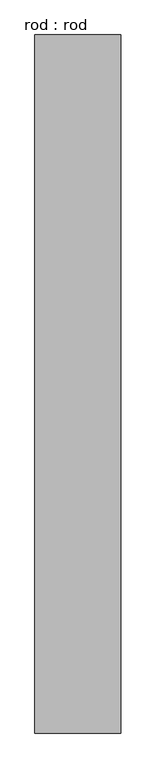
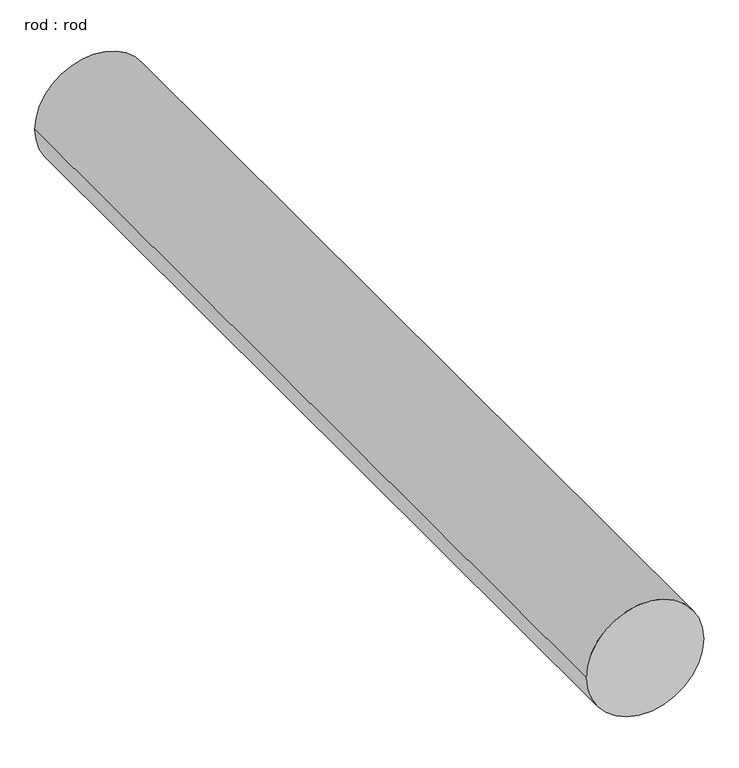
"""IFC4 building model written with IfcOpenShell, lengths in millimetres: proxy geometry, rod : rod."""

from ifc_helpers import new_model, si_unit, point, frame, frame_2d, origin, place, context, project, spatial, circle_curve, trimmed, segment, composite_curve, outline, extrude, source, transform, mapped, element, save


def rod_rod_cc77db4c(model_context):
    return source(origin(), model_context, "Body", "SweptSolid", [
        extrude(outline(composite_curve([segment(trimmed(circle_curve(frame_2d((0.0108462, 0.0)), 200.0), [point((0.0108462, 200.0))], [point((0.0108462, -200.0))], False, "CARTESIAN"), True, "CONTINUOUS"), segment(trimmed(circle_curve(frame_2d((0.0108462, 0.0)), 200.0), [point((0.0108462, -200.0))], [point((0.0108462, 200.0))], False, "CARTESIAN"), True, "CONTINUOUS")], self_intersect=False)), frame((0.0, 2464.1571868, 0.0), z_axis=(0.0, 1.0, 0.0), x_axis=(0.0, 0.0, 1.0)), (0.0, 0.0, 1.0), 3257.1428571),
    ])


if __name__ == "__main__":
    model = new_model("IFC4")
    model_context = context("Model", 3, world=origin())
    ifc_project = project(units=[si_unit("LENGTHUNIT", "METRE", prefix="MILLI")], contexts=[model_context])
    site = spatial("IfcSite", under=ifc_project)
    building = spatial("IfcBuilding", under=site)
    placement = place(None, origin())
    rod_rod_shape = rod_rod_cc77db4c(model_context)
    element("IfcBuildingElementProxy", 1, Name="rod : rod", ObjectType="rod : rod", at=placement, inside=building, context=model_context, shape_type="MappedRepresentation", body=[
        mapped(rod_rod_shape, transform((0.0, 0.0, 0.0), x_axis=(1.0, 0.0, 0.0), y_axis=(0.0, 1.0, 0.0), z_axis=(0.0, 0.0, 1.0))),
    ])
    save(model, "model.ifc")

# Revit data of these elements
# Type "rod : rod"
#   Default Elevation = 0
